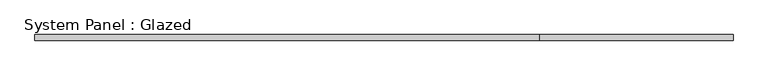
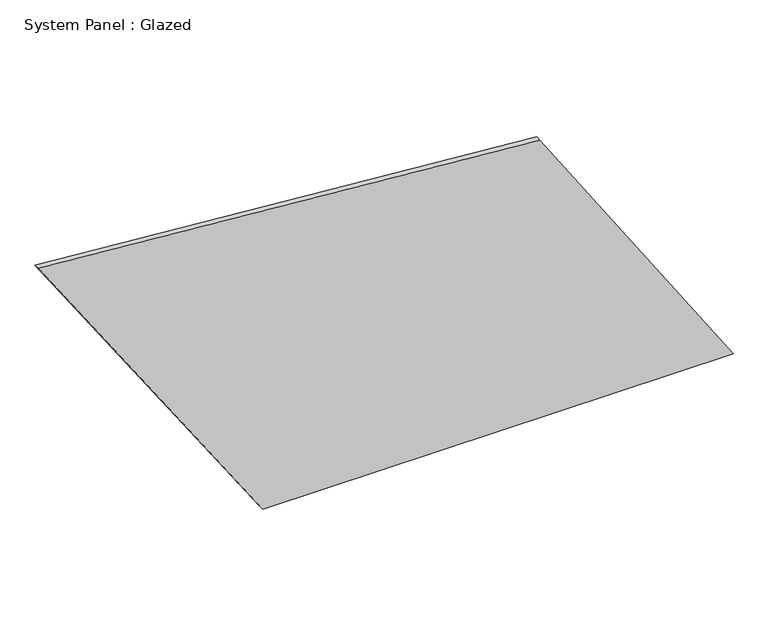
"""IFC4 building model written with IfcOpenShell, lengths in millimetres: plate geometry, System Panel : Glazed."""

from ifc_helpers import new_model, si_unit, frame, origin, place, context, project, spatial, polyline, outline, extrude, source, transform, mapped, element, save


def system_panel_glazed_d730aceb(model_context):
    return source(origin(), model_context, "Body", "SweptSolid", [
        extrude(outline(polyline([(0.0, -550.0394522), (0.0, 1558.5449962), (1315.8419208, 692.312148), (1496.3282928, -1558.5449962), (0.0, -550.0394522)])), frame((0.0, -49.5, 0.0), z_axis=(0.0, 1.0, 0.0), x_axis=(0.0, 0.0, 1.0)), (0.0, 0.0, 1.0), 25.0),
    ])


if __name__ == "__main__":
    model = new_model("IFC4")
    model_context = context("Model", 3, world=origin())
    ifc_project = project(units=[si_unit("LENGTHUNIT", "METRE", prefix="MILLI")], contexts=[model_context])
    site = spatial("IfcSite", under=ifc_project)
    building = spatial("IfcBuilding", under=site)
    placement = place(None, origin())
    system_panel_glazed_shape = system_panel_glazed_d730aceb(model_context)
    element("IfcPlate", 1, ObjectType="System Panel : Glazed", at=placement, inside=building, context=model_context, shape_type="MappedRepresentation", body=[
        mapped(system_panel_glazed_shape, transform((0.0, 0.0, 0.0), x_axis=(1.0, 0.0, 0.0), y_axis=(0.0, 1.0, 0.0), z_axis=(0.0, 0.0, 1.0))),
    ])
    save(model, "model.ifc")

# Revit data of these elements
# Element 1 (IfcPlate, "System Panel : Glazed")
#   Materials on its faces: "Glass, Clear Glazing"
# Materials
#   "Glass, Clear Glazing": class "Glass", colour RGB 247 249 248, transparency 0.85, Description = "Clear glazing", Cost = 0
